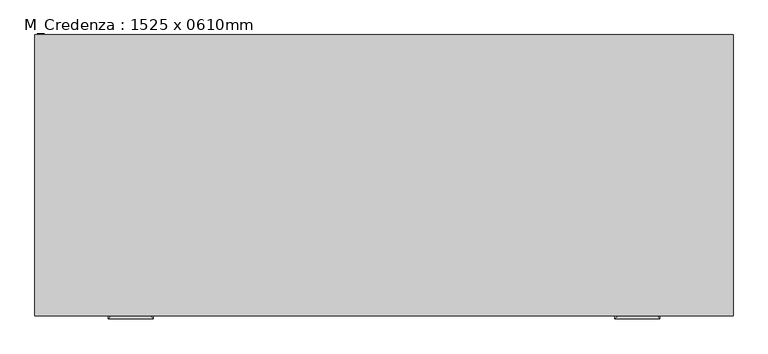
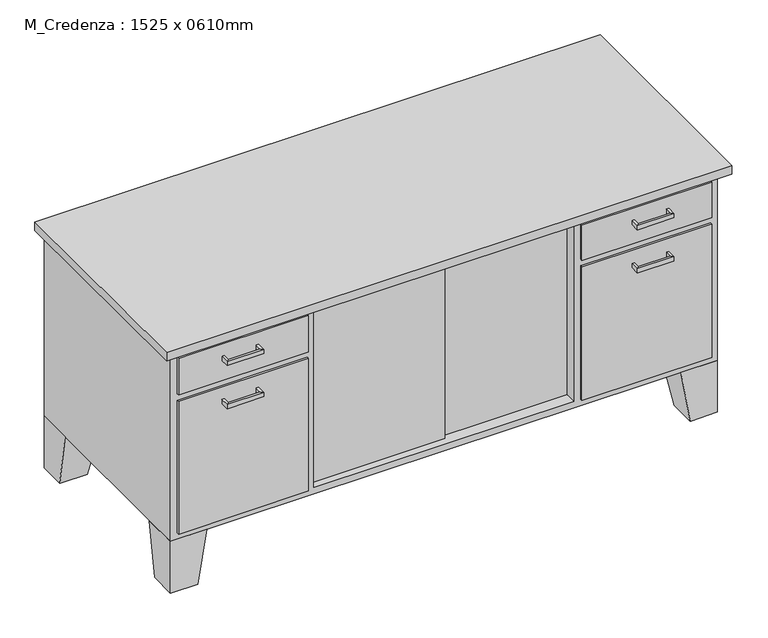
"""IFC4 building model written with IfcOpenShell, lengths in millimetres: furniture geometry, M_Credenza : 1525 x 0610mm."""

from ifc_helpers import new_model, si_unit, frame, origin, place, context, project, spatial, polyline, outline, extrude, faceted_brep, source, transform, mapped, element, save


def m_credenza_1525_x_0610mm_b960e448(model_context):
    return source(origin(), model_context, "Body", "SolidModel", [
        extrude(outline(polyline([(455.7523176, -267.0714583), (46.8442623, -267.0714583), (46.8442623, -254.7714583), (455.7523176, -254.7714583), (455.7523176, -267.0714583)])), frame((0.0, 0.0, 171.45), z_axis=(0.0, 0.0, 1.0), x_axis=(1.0, 0.0, 0.0)), (0.0, 0.0, 1.0), 518.1),
        extrude(outline(polyline([(73.6254475, -279.7714583), (-302.6557377, -279.7714583), (-302.6557377, -267.0714583), (73.6254475, -267.0714583), (73.6254475, -279.7714583)])), frame((0.0, 0.0, 171.45), z_axis=(0.0, 0.0, 1.0), x_axis=(1.0, 0.0, 0.0)), (0.0, 0.0, 1.0), 518.1),
        faceted_brep([(720.4442623, 309.5803279, 152.4), (720.4442623, 207.9803279, 152.4), (822.0442623, 207.9803279, 152.4), (822.0442623, 309.5803279, 152.4), (745.8442623, 309.5803279, 0.0), (822.0442623, 309.5803279, 0.0), (822.0442623, 233.3803279, 0.0), (745.8442623, 233.3803279, 0.0)], [[[0, 1, 2, 3]], [[4, 5, 6, 7]], [[4, 7, 1, 0]], [[7, 6, 2, 1]], [[6, 5, 3, 2]], [[5, 4, 0, 3]]]),
        extrude(outline(polyline([(802.9942623, -306.3696721), (440.7942623, -306.3696721), (440.7942623, -300.0196721), (802.9942623, -300.0196721), (802.9942623, -306.3696721)])), frame((0.0, 0.0, 584.2), z_axis=(0.0, 0.0, 1.0), x_axis=(1.0, 0.0, 0.0)), (0.0, 0.0, 1.0), 105.35),
        extrude(outline(polyline([(802.9942623, -306.3696721), (440.7942623, -306.3696721), (440.7942623, -300.0196721), (802.9942623, -300.0196721), (802.9942623, -306.3696721)])), frame((0.0, 0.0, 171.45), z_axis=(0.0, 0.0, 1.0), x_axis=(1.0, 0.0, 0.0)), (0.0, 0.0, 1.0), 393.7),
        extrude(outline(polyline([(-321.7057377, -306.7696721), (-683.9057377, -306.7696721), (-683.9057377, -300.4196721), (-321.7057377, -300.4196721), (-321.7057377, -306.7696721)])), frame((0.0, 0.0, 581.6), z_axis=(0.0, 0.0, 1.0), x_axis=(1.0, 0.0, 0.0)), (0.0, 0.0, 1.0), 107.95),
        extrude(outline(polyline([(-321.7057377, -306.7696721), (-683.9057377, -306.7696721), (-683.9057377, -300.4196721), (-321.7057377, -300.4196721), (-321.7057377, -306.7696721)])), frame((0.0, 0.0, 171.45), z_axis=(0.0, 0.0, 1.0), x_axis=(1.0, 0.0, 0.0)), (0.0, 0.0, 1.0), 391.1),
        faceted_brep([(-601.3557377, -300.4196721, 152.4), (-601.3557377, -198.8196721, 152.4), (-702.9557377, -198.8196721, 152.4), (-702.9557377, -300.4196721, 152.4), (-626.7557377, -300.4196721, 0.0), (-702.9557377, -300.4196721, 0.0), (-702.9557377, -224.2196721, 0.0), (-626.7557377, -224.2196721, 0.0)], [[[0, 1, 2, 3]], [[4, 5, 6, 7]], [[4, 7, 1, 0]], [[7, 6, 2, 1]], [[6, 5, 3, 2]], [[5, 4, 0, 3]]]),
        faceted_brep([(-601.3557377, 309.5803279, 152.4), (-702.9557377, 309.5803279, 152.4), (-702.9557377, 207.9803279, 152.4), (-601.3557377, 207.9803279, 152.4), (-626.7557377, 309.5803279, 0.0), (-626.7557377, 233.3803279, 0.0), (-702.9557377, 233.3803279, 0.0), (-702.9557377, 309.5803279, 0.0)], [[[0, 1, 2, 3]], [[4, 5, 6, 7]], [[4, 7, 1, 0]], [[7, 6, 2, 1]], [[6, 5, 3, 2]], [[5, 4, 0, 3]]]),
        faceted_brep([(720.4442623, -300.4196721, 152.4), (822.0442623, -300.4196721, 152.4), (822.0442623, -198.8196721, 152.4), (720.4442623, -198.8196721, 152.4), (745.8442623, -300.4196721, 0.0), (745.8442623, -224.2196721, 0.0), (822.0442623, -224.2196721, 0.0), (822.0442623, -300.4196721, 0.0)], [[[0, 1, 2, 3]], [[4, 5, 6, 7]], [[4, 7, 1, 0]], [[7, 6, 2, 1]], [[6, 5, 3, 2]], [[5, 4, 0, 3]]]),
        faceted_brep([(822.0442623, 309.5803279, 708.6), (-702.9557377, 309.5803279, 708.6), (-702.9557377, -300.4196721, 708.6), (822.0442623, -300.4196721, 708.6), (822.0442623, 309.5803279, 152.4), (822.0442623, -300.4196721, 152.4), (-702.9557377, -300.4196721, 152.4), (-702.9557377, 309.5803279, 152.4), (-302.6557377, -300.4196721, 689.55), (421.7442623, -300.4196721, 689.55), (421.7442623, -300.4196721, 171.45), (-302.6557377, -300.4196721, 171.45), (421.7442623, 290.3303279, 689.55), (-302.6557377, 290.3303279, 689.55), (-302.6557377, 290.3303279, 171.45), (421.7442623, 290.3303279, 171.45)], [[[0, 1, 2, 3]], [[4, 5, 6, 7]], [[1, 0, 4, 7]], [[2, 1, 7, 6]], [[3, 2, 6, 5], [8, 9, 10, 11]], [[0, 3, 5, 4]], [[12, 13, 14, 15]], [[13, 12, 9, 8]], [[14, 13, 8, 11]], [[15, 14, 11, 10]], [[12, 15, 10, 9]]]),
        extrude(outline(polyline([(847.4442623, 309.5803279), (847.4442623, -325.8196721), (-728.3557377, -325.8196721), (-728.3557377, 309.5803279), (847.4442623, 309.5803279)])), frame((0.0, 0.0, 708.6), z_axis=(0.0, 0.0, 1.0), x_axis=(1.0, 0.0, 0.0)), (0.0, 0.0, 1.0), 25.4),
        faceted_brep([(-556.7807377, -306.7696721, 527.05), (-556.7807377, -306.7696721, 514.35), (-563.1307377, -306.7696721, 514.35), (-563.1307377, -306.7696721, 527.05), (-556.7807377, -325.8196721, 527.05), (-556.7807377, -325.8196721, 514.35), (-563.1307377, -332.1696721, 514.35), (-563.1307377, -332.1696721, 527.05), (-467.8807377, -325.8196721, 527.05), (-467.8807377, -325.8196721, 514.35), (-461.5307377, -332.1696721, 514.35), (-461.5307377, -332.1696721, 527.05), (-467.8807377, -306.7696721, 527.05), (-461.5307377, -306.7696721, 527.05), (-461.5307377, -306.7696721, 514.35), (-467.8807377, -306.7696721, 514.35)], [[[0, 1, 2, 3]], [[1, 0, 4, 5]], [[2, 1, 5, 6]], [[3, 2, 6, 7]], [[0, 3, 7, 4]], [[5, 4, 8, 9]], [[6, 5, 9, 10]], [[7, 6, 10, 11]], [[4, 7, 11, 8]], [[12, 13, 14, 15]], [[9, 8, 12, 15]], [[10, 9, 15, 14]], [[11, 10, 14, 13]], [[8, 11, 13, 12]]]),
        faceted_brep([(-556.7807377, -306.7696721, 654.05), (-556.7807377, -306.7696721, 641.35), (-563.1307377, -306.7696721, 641.35), (-563.1307377, -306.7696721, 654.05), (-556.7807377, -325.8196721, 654.05), (-556.7807377, -325.8196721, 641.35), (-563.1307377, -332.1696721, 641.35), (-563.1307377, -332.1696721, 654.05), (-467.8807377, -325.8196721, 654.05), (-467.8807377, -325.8196721, 641.35), (-461.5307377, -332.1696721, 641.35), (-461.5307377, -332.1696721, 654.05), (-467.8807377, -306.7696721, 654.05), (-461.5307377, -306.7696721, 654.05), (-461.5307377, -306.7696721, 641.35), (-467.8807377, -306.7696721, 641.35)], [[[0, 1, 2, 3]], [[1, 0, 4, 5]], [[2, 1, 5, 6]], [[3, 2, 6, 7]], [[0, 3, 7, 4]], [[5, 4, 8, 9]], [[6, 5, 9, 10]], [[7, 6, 10, 11]], [[4, 7, 11, 8]], [[12, 13, 14, 15]], [[9, 8, 12, 15]], [[10, 9, 15, 14]], [[11, 10, 14, 13]], [[8, 11, 13, 12]]]),
        faceted_brep([(586.9692623, -306.7696721, 654.1373112), (586.9692623, -306.7696721, 641.4373112), (580.6192623, -306.7696721, 641.4373112), (580.6192623, -306.7696721, 654.1373112), (586.9692623, -325.8196721, 654.1373112), (586.9692623, -325.8196721, 641.4373112), (580.6192623, -332.1696721, 641.4373112), (580.6192623, -332.1696721, 654.1373112), (675.8692623, -325.8196721, 654.1373112), (675.8692623, -325.8196721, 641.4373112), (682.2192623, -332.1696721, 641.4373112), (682.2192623, -332.1696721, 654.1373112), (675.8692623, -306.7696721, 654.1373112), (682.2192623, -306.7696721, 654.1373112), (682.2192623, -306.7696721, 641.4373112), (675.8692623, -306.7696721, 641.4373112)], [[[0, 1, 2, 3]], [[1, 0, 4, 5]], [[2, 1, 5, 6]], [[3, 2, 6, 7]], [[0, 3, 7, 4]], [[5, 4, 8, 9]], [[6, 5, 9, 10]], [[7, 6, 10, 11]], [[4, 7, 11, 8]], [[12, 13, 14, 15]], [[9, 8, 12, 15]], [[10, 9, 15, 14]], [[11, 10, 14, 13]], [[8, 11, 13, 12]]]),
        faceted_brep([(586.9692623, -306.7696721, 527.05), (586.9692623, -306.7696721, 514.35), (580.6192623, -306.7696721, 514.35), (580.6192623, -306.7696721, 527.05), (586.9692623, -325.8196721, 527.05), (586.9692623, -325.8196721, 514.35), (580.6192623, -332.1696721, 514.35), (580.6192623, -332.1696721, 527.05), (675.8692623, -325.8196721, 527.05), (675.8692623, -325.8196721, 514.35), (682.2192623, -332.1696721, 514.35), (682.2192623, -332.1696721, 527.05), (675.8692623, -306.7696721, 527.05), (682.2192623, -306.7696721, 527.05), (682.2192623, -306.7696721, 514.35), (675.8692623, -306.7696721, 514.35)], [[[0, 1, 2, 3]], [[1, 0, 4, 5]], [[2, 1, 5, 6]], [[3, 2, 6, 7]], [[0, 3, 7, 4]], [[5, 4, 8, 9]], [[6, 5, 9, 10]], [[7, 6, 10, 11]], [[4, 7, 11, 8]], [[12, 13, 14, 15]], [[9, 8, 12, 15]], [[10, 9, 15, 14]], [[11, 10, 14, 13]], [[8, 11, 13, 12]]]),
    ])


if __name__ == "__main__":
    model = new_model("IFC4")
    model_context = context("Model", 3, world=origin())
    ifc_project = project(units=[si_unit("LENGTHUNIT", "METRE", prefix="MILLI")], contexts=[model_context])
    site = spatial("IfcSite", under=ifc_project)
    building = spatial("IfcBuilding", under=site)
    placement = place(None, origin())
    m_credenza_1525_x_0610mm_shape = m_credenza_1525_x_0610mm_b960e448(model_context)
    element("IfcFurniture", 1, ObjectType="M_Credenza : 1525 x 0610mm", at=placement, inside=building, context=model_context, shape_type="MappedRepresentation", body=[
        mapped(m_credenza_1525_x_0610mm_shape, transform((0.0, 0.0, 0.0), x_axis=(1.0, 0.0, 0.0), y_axis=(0.0, 1.0, 0.0), z_axis=(0.0, 0.0, 1.0))),
    ])
    save(model, "model.ifc")

# Revit data of these elements
# Type "M_Credenza : 1525 x 0610mm"
#   Depth = 0.61 m
#   Height = 0.734 m
#   Width = 1.525 m
#   Desk-Body = Laminate, Ivory, Matte
#   Handle/Leg Material = Steel, Chrome Plated
#   Top Material = Cherry
#   Default Elevation = 0
# Element 1 (IfcFurniture, "M_Credenza : 1525 x 0610mm")
#   Materials on its faces: "Steel, Chrome Plated", "Laminate, Ivory, Matte", "Cherry"
# Materials
#   "Laminate, Ivory, Matte": class "Plastic", colour RGB 247 247 229, transparency 0, Description = "Plastic Laminate - Ivory, Matte", Cost = 0
#   "Steel, Chrome Plated": class "Metal", colour RGB 244 244 244, transparency 0, Description = "Chromiuim plated steel", Cost = 0
#   "Cherry": class "Wood", colour RGB 157 77 38, transparency 0, Description = "Prunus Serotina", Cost = 0
